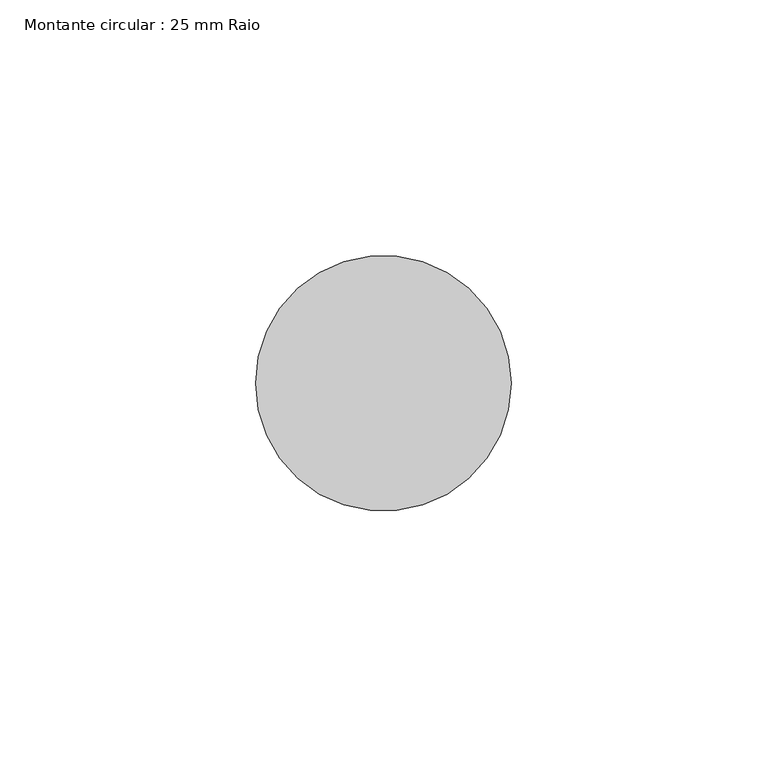
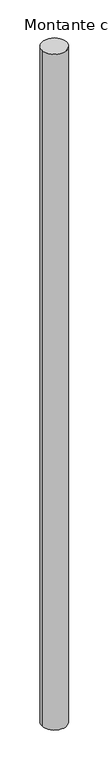
"""IFC4 building model written with IfcOpenShell, lengths in millimetres: member geometry, Montante circular : 25 mm Raio."""

from ifc_helpers import new_model, si_unit, point, frame, origin, origin_2d, place, context, project, spatial, circle_curve, trimmed, segment, composite_curve, outline, extrude, source, transform, mapped, element, save


def montante_circular_25_mm_raio_4202f854(model_context):
    return source(origin(), model_context, "Body", "SweptSolid", [
        extrude(outline(composite_curve([segment(trimmed(circle_curve(origin_2d(), 25.0), [point((25.0, 0.0))], [point((-25.0, 0.0))], False, "CARTESIAN"), True, "CONTINUOUS"), segment(trimmed(circle_curve(origin_2d(), 25.0), [point((-25.0, 0.0))], [point((25.0, 0.0))], False, "CARTESIAN"), True, "CONTINUOUS")], self_intersect=False)), frame((0.0, 0.0, -1431.9597241), z_axis=(0.0, 0.0, 1.0), x_axis=(1.0, 0.0, 0.0)), (0.0, 0.0, 1.0), 1431.9597241),
    ])


if __name__ == "__main__":
    model = new_model("IFC4")
    model_context = context("Model", 3, world=origin())
    ifc_project = project(units=[si_unit("LENGTHUNIT", "METRE", prefix="MILLI")], contexts=[model_context])
    site = spatial("IfcSite", under=ifc_project)
    building = spatial("IfcBuilding", under=site)
    placement = place(None, origin())
    montante_circular_25_mm_raio_shape = montante_circular_25_mm_raio_4202f854(model_context)
    element("IfcMember", 1, ObjectType="Montante circular : 25 mm Raio", at=placement, inside=building, context=model_context, shape_type="MappedRepresentation", body=[
        mapped(montante_circular_25_mm_raio_shape, transform((0.0, 0.0, 0.0), x_axis=(1.0, 0.0, 0.0), y_axis=(0.0, 1.0, 0.0), z_axis=(0.0, 0.0, 1.0))),
    ])
    save(model, "model.ifc")

# Revit data of these elements
# Type "Montante circular : 25 mm Raio"
#   built-in parameter 1007350 = 0.082021 (stored number, unit not read)
# Element 1 (IfcMember, "Montante circular : 25 mm Raio")
#   Materials on its faces: "Alumín."
# Materials
#   "Alumín.": class "Metal", colour RGB 247 247 247, transparency 0, Description = "Alumín. 6061", Cost = 0
